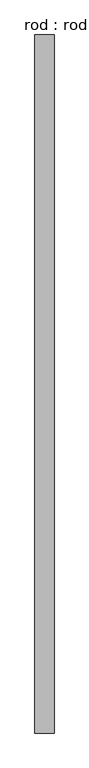
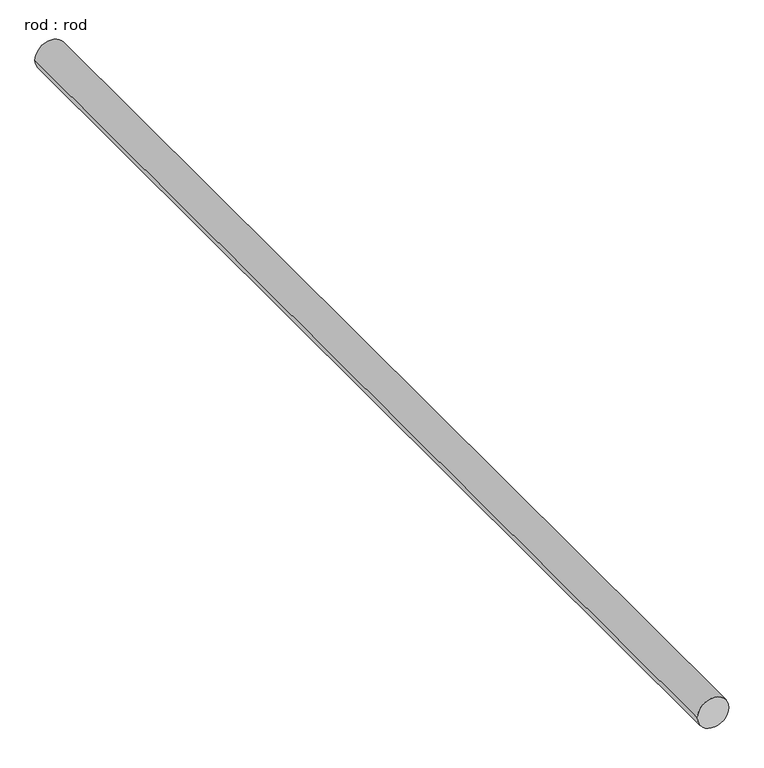
"""IFC4 building model written with IfcOpenShell, lengths in millimetres: proxy geometry, rod : rod."""

from ifc_helpers import new_model, si_unit, point, frame, frame_2d, origin, place, context, project, spatial, circle_curve, trimmed, segment, composite_curve, outline, extrude, source, transform, mapped, element, save


def rod_rod_a6798ba2(model_context):
    return source(origin(), model_context, "Body", "SweptSolid", [
        extrude(outline(composite_curve([segment(trimmed(circle_curve(frame_2d((0.0108462, 0.0)), 200.0), [point((0.0108462, 200.0))], [point((0.0108462, -200.0))], False, "CARTESIAN"), True, "CONTINUOUS"), segment(trimmed(circle_curve(frame_2d((0.0108462, 0.0)), 200.0), [point((0.0108462, -200.0))], [point((0.0108462, 200.0))], False, "CARTESIAN"), True, "CONTINUOUS")], self_intersect=False)), frame((0.0, -3218.0458197, 0.0), z_axis=(0.0, 1.0, 0.0), x_axis=(0.0, 0.0, 1.0)), (0.0, 0.0, 1.0), 14621.54887),
    ])


if __name__ == "__main__":
    model = new_model("IFC4")
    model_context = context("Model", 3, world=origin())
    ifc_project = project(units=[si_unit("LENGTHUNIT", "METRE", prefix="MILLI")], contexts=[model_context])
    site = spatial("IfcSite", under=ifc_project)
    building = spatial("IfcBuilding", under=site)
    placement = place(None, origin())
    rod_rod_shape = rod_rod_a6798ba2(model_context)
    element("IfcBuildingElementProxy", 1, Name="rod : rod", ObjectType="rod : rod", at=placement, inside=building, context=model_context, shape_type="MappedRepresentation", body=[
        mapped(rod_rod_shape, transform((0.0, 0.0, 0.0), x_axis=(1.0, 0.0, 0.0), y_axis=(0.0, 1.0, 0.0), z_axis=(0.0, 0.0, 1.0))),
    ])
    save(model, "model.ifc")

# Revit data of these elements
# Type "rod : rod"
#   Default Elevation = 0
